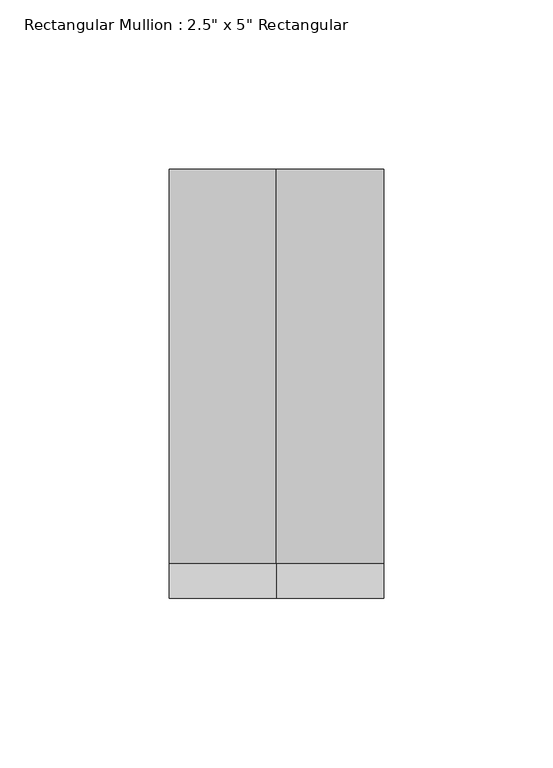
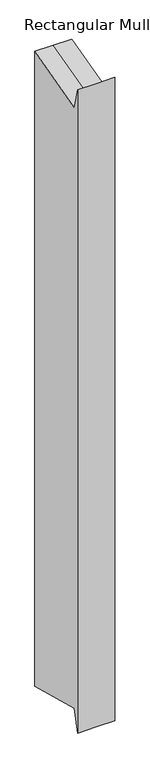
"""IFC4 building model written with IfcOpenShell, lengths in millimetres: member geometry."""

import ifcopenshell
import ifcopenshell.guid

model = None  # the IFC model being written
_history = None  # IfcOwnerHistory: only IFC2X3 demands one
_inside = {}  # id of a spatial element -> (the spatial element, [elements in it])
_under = {}  # id of a project, library or spatial element -> (it, [spatial elements below it])
_declared = {}  # id of a project -> (the project, [libraries it declares])
_typed = {}  # id of a type object -> (the type object, [elements of that type])
_made_of = {}  # id of a material, layer set ... -> (it, [elements and type objects made of it])


def new_model(schema):
    """Start an empty IFC model of exactly this schema.

    Asked for "IFC4X3", IfcOpenShell would pick the latest addendum, in which some entities
    have other attributes; the version numbers below select the first issue.
    IFC2X3 requires an IfcOwnerHistory on every rooted entity: one is made here for all.
    """
    global model, _history
    if schema == "IFC4X3":
        model = ifcopenshell.file(schema_version=(4, 3, 0, 0))
    else:
        model = ifcopenshell.file(schema=schema)
    _inside.clear()
    _under.clear()
    _declared.clear()
    _typed.clear()
    _made_of.clear()
    _history = None
    if model.schema == "IFC2X3":
        org = make("IfcOrganization", Name="unknown")
        user = make(
            "IfcPersonAndOrganization",
            ThePerson=make("IfcPerson", FamilyName="unknown"),
            TheOrganization=org,
        )
        app = make(
            "IfcApplication",
            ApplicationDeveloper=org,
            Version="unknown",
            ApplicationFullName="unknown",
            ApplicationIdentifier="unknown",
        )
        _history = make(
            "IfcOwnerHistory",
            OwningUser=user,
            OwningApplication=app,
            ChangeAction="ADDED",
            CreationDate=0,
        )
    return model


def make(cls, **values):
    """One entity of the class cls with the attributes given. An attribute that is None is left unset."""
    return model.create_entity(
        cls, **{name: value for name, value in values.items() if value is not None}
    )


def rooted(cls, **values):
    """An entity with a GlobalId (a new one), such as an element, a storey or a relation."""
    return make(cls, GlobalId=ifcopenshell.guid.new(), OwnerHistory=_history, **values)


def si_unit(unit_type, name, prefix=None):
    """IfcSIUnit, for example si_unit("LENGTHUNIT", "METRE", prefix="MILLI")."""
    return make("IfcSIUnit", UnitType=unit_type, Prefix=prefix, Name=name)


def assignment(units):
    """IfcUnitAssignment: the units of a project."""
    return None if units is None else make("IfcUnitAssignment", Units=units)


def point(xyz):
    """IfcCartesianPoint."""
    return None if xyz is None else make("IfcCartesianPoint", Coordinates=xyz)


def direction(xyz):
    """IfcDirection."""
    return None if xyz is None else make("IfcDirection", DirectionRatios=xyz)


def frame(location, z_axis=None, x_axis=None):
    """IfcAxis2Placement3D, a coordinate frame: its origin and axes. An axis left out is left unset."""
    return make(
        "IfcAxis2Placement3D",
        Location=point(location),
        Axis=direction(z_axis),
        RefDirection=direction(x_axis),
    )


def origin():
    """The frame at (0, 0, 0) with its axes left unset."""
    return frame((0.0, 0.0, 0.0))


def place(relative_to, where):
    """IfcLocalPlacement: puts the frame where relative to a parent placement (None: the world)."""
    return make(
        "IfcLocalPlacement", PlacementRelTo=relative_to, RelativePlacement=where
    )


def context(
    kind, dimensions, precision=None, world=None, true_north=None, identifier=None
):
    """IfcGeometricRepresentationContext, for example the 3D "Model" context."""
    return make(
        "IfcGeometricRepresentationContext",
        ContextIdentifier=identifier,
        ContextType=kind,
        CoordinateSpaceDimension=dimensions,
        Precision=precision,
        WorldCoordinateSystem=world,
        TrueNorth=true_north,
    )


def project(units=None, contexts=None):
    """IfcProject with its units and contexts."""
    return rooted(
        "IfcProject",
        Name="project",
        RepresentationContexts=contexts,
        UnitsInContext=assignment(units),
    )


def spatial(cls, under=None, at=None, **own):
    """A site, building, storey or space (cls), placed at a placement, below another one or the project."""
    s = rooted(cls, ObjectPlacement=at, **own)
    if under is not None:
        _under.setdefault(under.id(), (under, []))[1].append(s)
    return s


def faces_of(points, faces, orient=None, outer=None):
    """IfcFace entities. A face is a list of loops; a loop is a list of indices into points, from 0.

    orient and outer hold one flag for each loop. By default every Orientation is true, the
    first loop of a face is its IfcFaceOuterBound and the others are IfcFaceBound.
    """
    made = []
    for i, loops in enumerate(faces):
        bounds = []
        for j, loop in enumerate(loops):
            is_outer = j == 0 if outer is None else outer[i][j]
            bounds.append(
                make(
                    "IfcFaceOuterBound" if is_outer else "IfcFaceBound",
                    Bound=make("IfcPolyLoop", Polygon=[points[k] for k in loop]),
                    Orientation=True if orient is None else orient[i][j],
                )
            )
        made.append(make("IfcFace", Bounds=bounds))
    return made


def faceted_brep(points, faces, orient=None, outer=None, voids=None):
    """IfcFacetedBrep: a solid bounded by flat faces; with voids (closed shells), ...WithVoids."""
    shared = [point(p) for p in points]
    hull = make("IfcClosedShell", CfsFaces=faces_of(shared, faces, orient, outer))
    if voids is None:
        return make("IfcFacetedBrep", Outer=hull)
    return make(
        "IfcFacetedBrepWithVoids",
        Outer=hull,
        Voids=[
            make(cls, CfsFaces=faces_of(shared, fs, o, b)) for cls, fs, o, b in voids
        ],
    )


def shape(context_of_items, identifier, shape_type, items):
    """IfcShapeRepresentation: the items that make up one representation, for example the "Body"."""
    return make(
        "IfcShapeRepresentation",
        ContextOfItems=context_of_items,
        RepresentationIdentifier=identifier,
        RepresentationType=shape_type,
        Items=items,
    )


def source(mapping_origin, context_of_items, identifier, shape_type, items):
    """IfcRepresentationMap: a shape defined once, which mapped items show again and again."""
    return make(
        "IfcRepresentationMap",
        MappingOrigin=mapping_origin,
        MappedRepresentation=shape(context_of_items, identifier, shape_type, items),
    )


def transform(
    local_origin,
    x_axis=None,
    y_axis=None,
    z_axis=None,
    scale=None,
    scale2=None,
    scale3=None,
    uniform=True,
):
    """IfcCartesianTransformationOperator3D, or its non-uniform kind. x_axis, y_axis, z_axis: its Axis1, 2, 3."""
    if uniform:
        return make(
            "IfcCartesianTransformationOperator3D",
            Axis1=direction(x_axis),
            Axis2=direction(y_axis),
            LocalOrigin=point(local_origin),
            Scale=scale,
            Axis3=direction(z_axis),
        )
    return make(
        "IfcCartesianTransformationOperator3DnonUniform",
        Axis1=direction(x_axis),
        Axis2=direction(y_axis),
        LocalOrigin=point(local_origin),
        Scale=scale,
        Axis3=direction(z_axis),
        Scale2=scale2,
        Scale3=scale3,
    )


def mapped(mapping_source, mapping_target):
    """IfcMappedItem: shows the shape of a source again, moved by a transform."""
    return make(
        "IfcMappedItem", MappingSource=mapping_source, MappingTarget=mapping_target
    )


def made_of(thing, what):
    """Note that an element or type object is made of a material, layer set ...; save() writes the relation."""
    if what is not None:
        _made_of.setdefault(what.id(), (what, []))[1].append(thing)
    return thing


def element(
    cls,
    number,
    at=None,
    inside=None,
    cuts=None,
    type_object=None,
    material=None,
    context=None,
    identifier="Body",
    shape_type=None,
    held_by="IfcProductDefinitionShape",
    body=None,
    shapes=None,
    **own,
):
    """One element of the class cls, such as IfcWall. Its Tag is "e" and its number.

    at: its placement. inside: the storey or other place that contains it. cuts: it is an
    opening in that element (IfcRelVoidsElement). A single representation is given by context,
    identifier, shape_type and body (its items); several are given by shapes. held_by: the class
    of the entity that holds the representations. save() writes the other relations.
    """
    e = rooted(cls, Tag="e%d" % number, ObjectPlacement=at, **own)
    if body is not None:
        shapes = [shape(context, identifier, shape_type, body)]
    if shapes is not None:
        e.Representation = make(held_by, Representations=shapes)
    if inside is not None:
        _inside.setdefault(inside.id(), (inside, []))[1].append(e)
    if cuts is not None:
        rooted(
            "IfcRelVoidsElement", RelatingBuildingElement=cuts, RelatedOpeningElement=e
        )
    if type_object is not None:
        _typed.setdefault(type_object.id(), (type_object, []))[1].append(e)
    return made_of(e, material)


def aggregate(whole, parts):
    """IfcRelAggregates: a whole, such as a stair, and the parts it consists of."""
    return rooted("IfcRelAggregates", RelatingObject=whole, RelatedObjects=parts)


def save(model, path):
    """Write the relations noted so far, then the file.

    IfcRelAggregates (storeys below a building ...), IfcRelContainedInSpatialStructure (elements
    in a storey), IfcRelDefinesByType, IfcRelAssociatesMaterial and IfcRelDeclares: one each for
    every whole, place, type object, material and project.
    """
    for whole, parts in _under.values():
        aggregate(whole, parts)
    for where, things in _inside.values():
        rooted(
            "IfcRelContainedInSpatialStructure",
            RelatedElements=things,
            RelatingStructure=where,
        )
    for kind, things in _typed.values():
        rooted("IfcRelDefinesByType", RelatedObjects=things, RelatingType=kind)
    for what, things in _made_of.values():
        rooted("IfcRelAssociatesMaterial", RelatedObjects=things, RelatingMaterial=what)
    for by, libraries in _declared.values():
        rooted("IfcRelDeclares", RelatingContext=by, RelatedDefinitions=libraries)
    model.write(path)


def member_b6263386(model_context):
    return source(origin(), model_context, "Body", "Brep", [
        faceted_brep([(-31.75, 63.5, 15.894755), (0.0, 63.5, 15.894755), (31.75, 63.5, 15.894755), (31.75, 63.5, -1135.7154292), (0.0, 63.5, -1135.7154292), (-31.75, 63.5, -1135.7154292), (-31.75, -63.5, 23.3900664), (-31.75, -53.1187853, -15.3531543), (-31.75, -53.1187853, -1104.4675199), (-31.75, -63.5, -1143.2107406), (31.75, -63.5, 23.3900664), (0.0, -63.5, 23.3900664), (0.0, -63.5, -1143.2107406), (31.75, -63.5, -1143.2107406), (31.75, -53.1187853, -15.3531543), (31.75, -53.1187853, -1104.4675199), (0.0, -53.1187853, -15.3531543), (0.0, -53.1187853, -1104.4675199)], [[[0, 1, 2, 3, 4, 5]], [[6, 7, 0, 5, 8, 9]], [[10, 11, 6, 9, 12, 13]], [[2, 14, 10, 13, 15, 3]], [[2, 1, 16, 14]], [[1, 0, 7, 16]], [[7, 6, 11, 16]], [[11, 10, 14, 16]], [[3, 15, 17, 4]], [[15, 13, 12, 17]], [[12, 9, 8, 17]], [[8, 5, 4, 17]]]),
    ])


if __name__ == "__main__":
    model = new_model("IFC4")
    model_context = context("Model", 3, world=origin())
    ifc_project = project(units=[si_unit("LENGTHUNIT", "METRE", prefix="MILLI")], contexts=[model_context])
    site = spatial("IfcSite", under=ifc_project)
    building = spatial("IfcBuilding", under=site)
    placement = place(None, origin())
    member_shape = member_b6263386(model_context)
    element("IfcMember", 1, ObjectType="Rectangular Mullion : 2.5\" x 5\" Rectangular", at=placement, inside=building, context=model_context, shape_type="MappedRepresentation", body=[
        mapped(member_shape, transform((0.0, 0.0, 0.0), x_axis=(1.0, 0.0, 0.0), y_axis=(0.0, 1.0, 0.0), z_axis=(0.0, 0.0, 1.0))),
    ])
    save(model, "model.ifc")

# Revit data of these elements
# Type "Rectangular Mullion : 2.5\" x 5\" Rectangular"
#   built-in parameter 1007304 = 0.416667 (stored number, unit not read)
#   built-in parameter 1007301 = 0.104167 (stored number, unit not read)
#   built-in parameter 1007300 = 0.104167 (stored number, unit not read)
# Element 1 (IfcMember, "Rectangular Mullion : 2.5\" x 5\" Rectangular")
#   Materials on its faces: "Aluminum"
# Materials
#   "Aluminum": class "Metal", colour RGB 247 247 247, transparency 0, Description = "Aluminum 6061", Cost = 0
